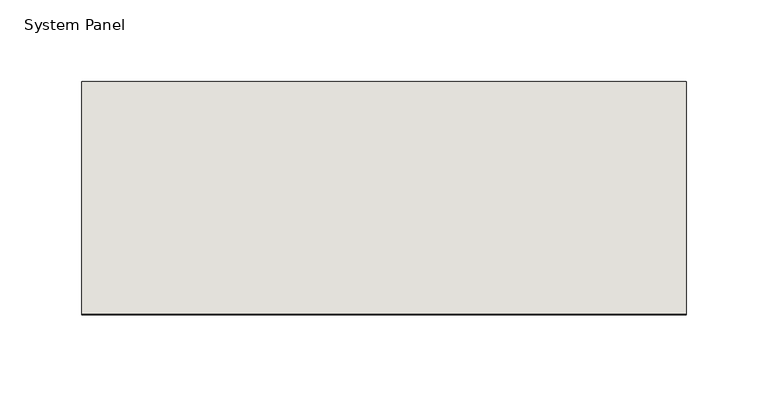
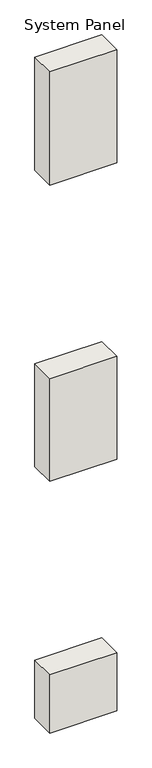
"""IFC4 building model written with IfcOpenShell, lengths in millimetres: wall geometry, System Panel : NLRS_21_CWP_hsb-vulling minerale wol 142 _gen_rsf."""

import ifcopenshell
import ifcopenshell.guid

model = None  # the IFC model being written
_history = None  # IfcOwnerHistory: only IFC2X3 demands one
_inside = {}  # id of a spatial element -> (the spatial element, [elements in it])
_under = {}  # id of a project, library or spatial element -> (it, [spatial elements below it])
_declared = {}  # id of a project -> (the project, [libraries it declares])
_typed = {}  # id of a type object -> (the type object, [elements of that type])
_made_of = {}  # id of a material, layer set ... -> (it, [elements and type objects made of it])


def new_model(schema):
    """Start an empty IFC model of exactly this schema.

    Asked for "IFC4X3", IfcOpenShell would pick the latest addendum, in which some entities
    have other attributes; the version numbers below select the first issue.
    IFC2X3 requires an IfcOwnerHistory on every rooted entity: one is made here for all.
    """
    global model, _history
    if schema == "IFC4X3":
        model = ifcopenshell.file(schema_version=(4, 3, 0, 0))
    else:
        model = ifcopenshell.file(schema=schema)
    _inside.clear()
    _under.clear()
    _declared.clear()
    _typed.clear()
    _made_of.clear()
    _history = None
    if model.schema == "IFC2X3":
        org = make("IfcOrganization", Name="unknown")
        user = make(
            "IfcPersonAndOrganization",
            ThePerson=make("IfcPerson", FamilyName="unknown"),
            TheOrganization=org,
        )
        app = make(
            "IfcApplication",
            ApplicationDeveloper=org,
            Version="unknown",
            ApplicationFullName="unknown",
            ApplicationIdentifier="unknown",
        )
        _history = make(
            "IfcOwnerHistory",
            OwningUser=user,
            OwningApplication=app,
            ChangeAction="ADDED",
            CreationDate=0,
        )
    return model


def make(cls, **values):
    """One entity of the class cls with the attributes given. An attribute that is None is left unset."""
    return model.create_entity(
        cls, **{name: value for name, value in values.items() if value is not None}
    )


def rooted(cls, **values):
    """An entity with a GlobalId (a new one), such as an element, a storey or a relation."""
    return make(cls, GlobalId=ifcopenshell.guid.new(), OwnerHistory=_history, **values)


def si_unit(unit_type, name, prefix=None):
    """IfcSIUnit, for example si_unit("LENGTHUNIT", "METRE", prefix="MILLI")."""
    return make("IfcSIUnit", UnitType=unit_type, Prefix=prefix, Name=name)


def assignment(units):
    """IfcUnitAssignment: the units of a project."""
    return None if units is None else make("IfcUnitAssignment", Units=units)


def point(xyz):
    """IfcCartesianPoint."""
    return None if xyz is None else make("IfcCartesianPoint", Coordinates=xyz)


def direction(xyz):
    """IfcDirection."""
    return None if xyz is None else make("IfcDirection", DirectionRatios=xyz)


def frame(location, z_axis=None, x_axis=None):
    """IfcAxis2Placement3D, a coordinate frame: its origin and axes. An axis left out is left unset."""
    return make(
        "IfcAxis2Placement3D",
        Location=point(location),
        Axis=direction(z_axis),
        RefDirection=direction(x_axis),
    )


def origin():
    """The frame at (0, 0, 0) with its axes left unset."""
    return frame((0.0, 0.0, 0.0))


def origin_with_axes():
    """The frame at (0, 0, 0) with the z axis (0, 0, 1) and the x axis (1, 0, 0) written out."""
    return frame((0.0, 0.0, 0.0), z_axis=(0.0, 0.0, 1.0), x_axis=(1.0, 0.0, 0.0))


def place(relative_to, where):
    """IfcLocalPlacement: puts the frame where relative to a parent placement (None: the world)."""
    return make(
        "IfcLocalPlacement", PlacementRelTo=relative_to, RelativePlacement=where
    )


def context(
    kind, dimensions, precision=None, world=None, true_north=None, identifier=None
):
    """IfcGeometricRepresentationContext, for example the 3D "Model" context."""
    return make(
        "IfcGeometricRepresentationContext",
        ContextIdentifier=identifier,
        ContextType=kind,
        CoordinateSpaceDimension=dimensions,
        Precision=precision,
        WorldCoordinateSystem=world,
        TrueNorth=true_north,
    )


def project(units=None, contexts=None):
    """IfcProject with its units and contexts."""
    return rooted(
        "IfcProject",
        Name="project",
        RepresentationContexts=contexts,
        UnitsInContext=assignment(units),
    )


def spatial(cls, under=None, at=None, **own):
    """A site, building, storey or space (cls), placed at a placement, below another one or the project."""
    s = rooted(cls, ObjectPlacement=at, **own)
    if under is not None:
        _under.setdefault(under.id(), (under, []))[1].append(s)
    return s


def polyline(points):
    """IfcPolyline through the points."""
    return make("IfcPolyline", Points=[point(p) for p in points])


def outline(outer, holes=None, kind="AREA"):
    """IfcArbitraryClosedProfileDef: a profile drawn as a closed curve; with holes, ...WithVoids."""
    if holes is None:
        return make("IfcArbitraryClosedProfileDef", ProfileType=kind, OuterCurve=outer)
    return make(
        "IfcArbitraryProfileDefWithVoids",
        ProfileType=kind,
        OuterCurve=outer,
        InnerCurves=holes,
    )


def extrude(swept, where, along, depth):
    """IfcExtrudedAreaSolid: the profile swept, set in the frame where, extruded along a direction by depth."""
    return make(
        "IfcExtrudedAreaSolid",
        SweptArea=swept,
        Position=where,
        ExtrudedDirection=direction(along),
        Depth=depth,
    )


def shape(context_of_items, identifier, shape_type, items):
    """IfcShapeRepresentation: the items that make up one representation, for example the "Body"."""
    return make(
        "IfcShapeRepresentation",
        ContextOfItems=context_of_items,
        RepresentationIdentifier=identifier,
        RepresentationType=shape_type,
        Items=items,
    )


def source(mapping_origin, context_of_items, identifier, shape_type, items):
    """IfcRepresentationMap: a shape defined once, which mapped items show again and again."""
    return make(
        "IfcRepresentationMap",
        MappingOrigin=mapping_origin,
        MappedRepresentation=shape(context_of_items, identifier, shape_type, items),
    )


def transform(
    local_origin,
    x_axis=None,
    y_axis=None,
    z_axis=None,
    scale=None,
    scale2=None,
    scale3=None,
    uniform=True,
):
    """IfcCartesianTransformationOperator3D, or its non-uniform kind. x_axis, y_axis, z_axis: its Axis1, 2, 3."""
    if uniform:
        return make(
            "IfcCartesianTransformationOperator3D",
            Axis1=direction(x_axis),
            Axis2=direction(y_axis),
            LocalOrigin=point(local_origin),
            Scale=scale,
            Axis3=direction(z_axis),
        )
    return make(
        "IfcCartesianTransformationOperator3DnonUniform",
        Axis1=direction(x_axis),
        Axis2=direction(y_axis),
        LocalOrigin=point(local_origin),
        Scale=scale,
        Axis3=direction(z_axis),
        Scale2=scale2,
        Scale3=scale3,
    )


def mapped(mapping_source, mapping_target):
    """IfcMappedItem: shows the shape of a source again, moved by a transform."""
    return make(
        "IfcMappedItem", MappingSource=mapping_source, MappingTarget=mapping_target
    )


def made_of(thing, what):
    """Note that an element or type object is made of a material, layer set ...; save() writes the relation."""
    if what is not None:
        _made_of.setdefault(what.id(), (what, []))[1].append(thing)
    return thing


def element(
    cls,
    number,
    at=None,
    inside=None,
    cuts=None,
    type_object=None,
    material=None,
    context=None,
    identifier="Body",
    shape_type=None,
    held_by="IfcProductDefinitionShape",
    body=None,
    shapes=None,
    **own,
):
    """One element of the class cls, such as IfcWall. Its Tag is "e" and its number.

    at: its placement. inside: the storey or other place that contains it. cuts: it is an
    opening in that element (IfcRelVoidsElement). A single representation is given by context,
    identifier, shape_type and body (its items); several are given by shapes. held_by: the class
    of the entity that holds the representations. save() writes the other relations.
    """
    e = rooted(cls, Tag="e%d" % number, ObjectPlacement=at, **own)
    if body is not None:
        shapes = [shape(context, identifier, shape_type, body)]
    if shapes is not None:
        e.Representation = make(held_by, Representations=shapes)
    if inside is not None:
        _inside.setdefault(inside.id(), (inside, []))[1].append(e)
    if cuts is not None:
        rooted(
            "IfcRelVoidsElement", RelatingBuildingElement=cuts, RelatedOpeningElement=e
        )
    if type_object is not None:
        _typed.setdefault(type_object.id(), (type_object, []))[1].append(e)
    return made_of(e, material)


def aggregate(whole, parts):
    """IfcRelAggregates: a whole, such as a stair, and the parts it consists of."""
    return rooted("IfcRelAggregates", RelatingObject=whole, RelatedObjects=parts)


def save(model, path):
    """Write the relations noted so far, then the file.

    IfcRelAggregates (storeys below a building ...), IfcRelContainedInSpatialStructure (elements
    in a storey), IfcRelDefinesByType, IfcRelAssociatesMaterial and IfcRelDeclares: one each for
    every whole, place, type object, material and project.
    """
    for whole, parts in _under.values():
        aggregate(whole, parts)
    for where, things in _inside.values():
        rooted(
            "IfcRelContainedInSpatialStructure",
            RelatedElements=things,
            RelatingStructure=where,
        )
    for kind, things in _typed.values():
        rooted("IfcRelDefinesByType", RelatedObjects=things, RelatingType=kind)
    for what, things in _made_of.values():
        rooted("IfcRelAssociatesMaterial", RelatedObjects=things, RelatingMaterial=what)
    for by, libraries in _declared.values():
        rooted("IfcRelDeclares", RelatingContext=by, RelatedDefinitions=libraries)
    model.write(path)


def system_panel_bba4faf4(model_context):
    return source(origin(), model_context, "Body", "SweptSolid", [
        extrude(outline(polyline([(184.5, -71.0), (-184.5, -71.0), (-184.5, 71.0), (184.5, 71.0), (184.5, -71.0)])), frame((0.0, 0.0, 3190.0), z_axis=(0.0, 0.0, 1.0), x_axis=(1.0, 0.0, 0.0)), (0.0, 0.0, 1.0), 659.0),
        extrude(outline(polyline([(184.5, -71.0), (-184.5, -71.0), (-184.5, 71.0), (184.5, 71.0), (184.5, -71.0)])), frame((0.0, 0.0, 1465.0), z_axis=(0.0, 0.0, 1.0), x_axis=(1.0, 0.0, 0.0)), (0.0, 0.0, 1.0), 599.0),
        extrude(outline(polyline([(184.5, -71.0), (-184.5, -71.0), (-184.5, 71.0), (184.5, 71.0), (184.5, -71.0)])), origin_with_axes(), (0.0, 0.0, 1.0), 339.0),
    ])


if __name__ == "__main__":
    model = new_model("IFC4")
    model_context = context("Model", 3, world=origin())
    ifc_project = project(units=[si_unit("LENGTHUNIT", "METRE", prefix="MILLI")], contexts=[model_context])
    site = spatial("IfcSite", under=ifc_project)
    building = spatial("IfcBuilding", under=site)
    placement = place(None, origin())
    system_panel_shape = system_panel_bba4faf4(model_context)
    element("IfcWall", 1, ObjectType="System Panel : NLRS_21_CWP_hsb-vulling minerale wol 142 _gen_rsf", at=placement, inside=building, context=model_context, shape_type="MappedRepresentation", body=[
        mapped(system_panel_shape, transform((0.0, 0.0, 0.0), x_axis=(1.0, 0.0, 0.0), y_axis=(0.0, 1.0, 0.0), z_axis=(0.0, 0.0, 1.0))),
    ])
    save(model, "model.ifc")

# Revit data of these elements
# Type "System Panel : NLRS_21_CWP_hsb-vulling minerale wol 142 _gen_rsf"
#   Type IfcGUID = "07M7mRoiH1CR8m_RSKIwpC"
#   Assembly Code = "21.23"
#   IfcExportAs = "IfcWall"
# Element 1 (IfcWall, "System Panel : NLRS_21_CWP_hsb-vulling minerale wol 142 _gen_rsf")
#   Materials on its faces: "NLRS_m1_isolatie minerale wol_gen_rsf"
# Materials
#   "NLRS_m1_isolatie minerale wol_gen_rsf": class "M - Anorganische materialen", colour RGB 200 200 140, transparency 0, Keynote = "m1", Manufacturer = "Revit Standards Foundation", URL = "www.revitstandards.org", Description = "isolatie minerale wol", Cost = 0
